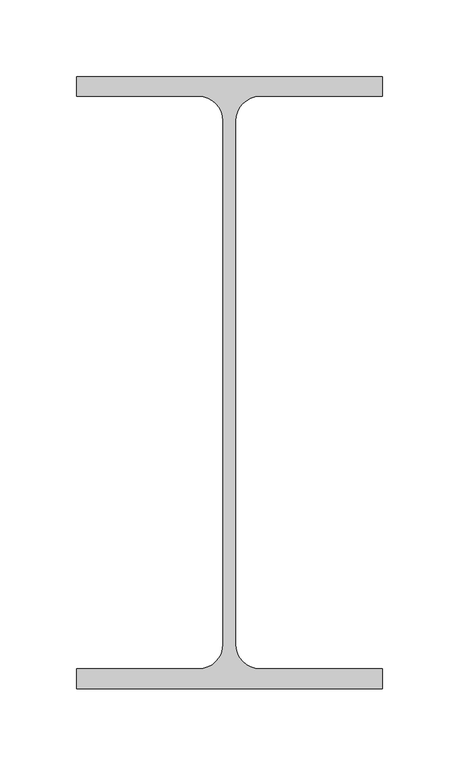
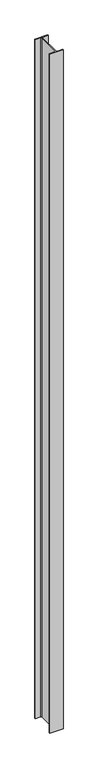
"""IFC4 building model written with IfcOpenShell, lengths in millimetres: column geometry, 0912_Steel Column_H_KSD3502 : H_SC_ASC_H-400x200x8x13."""

import ifcopenshell
import ifcopenshell.guid

model = None  # the IFC model being written
_history = None  # IfcOwnerHistory: only IFC2X3 demands one
_inside = {}  # id of a spatial element -> (the spatial element, [elements in it])
_under = {}  # id of a project, library or spatial element -> (it, [spatial elements below it])
_declared = {}  # id of a project -> (the project, [libraries it declares])
_typed = {}  # id of a type object -> (the type object, [elements of that type])
_made_of = {}  # id of a material, layer set ... -> (it, [elements and type objects made of it])


def new_model(schema):
    """Start an empty IFC model of exactly this schema.

    Asked for "IFC4X3", IfcOpenShell would pick the latest addendum, in which some entities
    have other attributes; the version numbers below select the first issue.
    IFC2X3 requires an IfcOwnerHistory on every rooted entity: one is made here for all.
    """
    global model, _history
    if schema == "IFC4X3":
        model = ifcopenshell.file(schema_version=(4, 3, 0, 0))
    else:
        model = ifcopenshell.file(schema=schema)
    _inside.clear()
    _under.clear()
    _declared.clear()
    _typed.clear()
    _made_of.clear()
    _history = None
    if model.schema == "IFC2X3":
        org = make("IfcOrganization", Name="unknown")
        user = make(
            "IfcPersonAndOrganization",
            ThePerson=make("IfcPerson", FamilyName="unknown"),
            TheOrganization=org,
        )
        app = make(
            "IfcApplication",
            ApplicationDeveloper=org,
            Version="unknown",
            ApplicationFullName="unknown",
            ApplicationIdentifier="unknown",
        )
        _history = make(
            "IfcOwnerHistory",
            OwningUser=user,
            OwningApplication=app,
            ChangeAction="ADDED",
            CreationDate=0,
        )
    return model


def make(cls, **values):
    """One entity of the class cls with the attributes given. An attribute that is None is left unset."""
    return model.create_entity(
        cls, **{name: value for name, value in values.items() if value is not None}
    )


def rooted(cls, **values):
    """An entity with a GlobalId (a new one), such as an element, a storey or a relation."""
    return make(cls, GlobalId=ifcopenshell.guid.new(), OwnerHistory=_history, **values)


def si_unit(unit_type, name, prefix=None):
    """IfcSIUnit, for example si_unit("LENGTHUNIT", "METRE", prefix="MILLI")."""
    return make("IfcSIUnit", UnitType=unit_type, Prefix=prefix, Name=name)


def assignment(units):
    """IfcUnitAssignment: the units of a project."""
    return None if units is None else make("IfcUnitAssignment", Units=units)


def point(xyz):
    """IfcCartesianPoint."""
    return None if xyz is None else make("IfcCartesianPoint", Coordinates=xyz)


def direction(xyz):
    """IfcDirection."""
    return None if xyz is None else make("IfcDirection", DirectionRatios=xyz)


def frame(location, z_axis=None, x_axis=None):
    """IfcAxis2Placement3D, a coordinate frame: its origin and axes. An axis left out is left unset."""
    return make(
        "IfcAxis2Placement3D",
        Location=point(location),
        Axis=direction(z_axis),
        RefDirection=direction(x_axis),
    )


def frame_2d(location, x_axis=None):
    """IfcAxis2Placement2D, a coordinate frame in the plane: its origin and x axis."""
    return make(
        "IfcAxis2Placement2D", Location=point(location), RefDirection=direction(x_axis)
    )


def origin():
    """The frame at (0, 0, 0) with its axes left unset."""
    return frame((0.0, 0.0, 0.0))


def place(relative_to, where):
    """IfcLocalPlacement: puts the frame where relative to a parent placement (None: the world)."""
    return make(
        "IfcLocalPlacement", PlacementRelTo=relative_to, RelativePlacement=where
    )


def context(
    kind, dimensions, precision=None, world=None, true_north=None, identifier=None
):
    """IfcGeometricRepresentationContext, for example the 3D "Model" context."""
    return make(
        "IfcGeometricRepresentationContext",
        ContextIdentifier=identifier,
        ContextType=kind,
        CoordinateSpaceDimension=dimensions,
        Precision=precision,
        WorldCoordinateSystem=world,
        TrueNorth=true_north,
    )


def project(units=None, contexts=None):
    """IfcProject with its units and contexts."""
    return rooted(
        "IfcProject",
        Name="project",
        RepresentationContexts=contexts,
        UnitsInContext=assignment(units),
    )


def spatial(cls, under=None, at=None, **own):
    """A site, building, storey or space (cls), placed at a placement, below another one or the project."""
    s = rooted(cls, ObjectPlacement=at, **own)
    if under is not None:
        _under.setdefault(under.id(), (under, []))[1].append(s)
    return s


def polyline(points):
    """IfcPolyline through the points."""
    return make("IfcPolyline", Points=[point(p) for p in points])


def circle_curve(where, radius):
    """IfcCircle in the frame where."""
    return make("IfcCircle", Position=where, Radius=radius)


def trimmed(basis, trim1, trim2, sense, master):
    """IfcTrimmedCurve: the piece of a basis curve between two trims."""
    return make(
        "IfcTrimmedCurve",
        BasisCurve=basis,
        Trim1=trim1,
        Trim2=trim2,
        SenseAgreement=sense,
        MasterRepresentation=master,
    )


def segment(curve, same_sense, transition):
    """IfcCompositeCurveSegment."""
    return make(
        "IfcCompositeCurveSegment",
        Transition=transition,
        SameSense=same_sense,
        ParentCurve=curve,
    )


def composite_curve(segments, self_intersect=None):
    """IfcCompositeCurve: segments joined end to end."""
    return make("IfcCompositeCurve", Segments=segments, SelfIntersect=self_intersect)


def outline(outer, holes=None, kind="AREA"):
    """IfcArbitraryClosedProfileDef: a profile drawn as a closed curve; with holes, ...WithVoids."""
    if holes is None:
        return make("IfcArbitraryClosedProfileDef", ProfileType=kind, OuterCurve=outer)
    return make(
        "IfcArbitraryProfileDefWithVoids",
        ProfileType=kind,
        OuterCurve=outer,
        InnerCurves=holes,
    )


def extrude(swept, where, along, depth):
    """IfcExtrudedAreaSolid: the profile swept, set in the frame where, extruded along a direction by depth."""
    return make(
        "IfcExtrudedAreaSolid",
        SweptArea=swept,
        Position=where,
        ExtrudedDirection=direction(along),
        Depth=depth,
    )


def shape(context_of_items, identifier, shape_type, items):
    """IfcShapeRepresentation: the items that make up one representation, for example the "Body"."""
    return make(
        "IfcShapeRepresentation",
        ContextOfItems=context_of_items,
        RepresentationIdentifier=identifier,
        RepresentationType=shape_type,
        Items=items,
    )


def source(mapping_origin, context_of_items, identifier, shape_type, items):
    """IfcRepresentationMap: a shape defined once, which mapped items show again and again."""
    return make(
        "IfcRepresentationMap",
        MappingOrigin=mapping_origin,
        MappedRepresentation=shape(context_of_items, identifier, shape_type, items),
    )


def transform(
    local_origin,
    x_axis=None,
    y_axis=None,
    z_axis=None,
    scale=None,
    scale2=None,
    scale3=None,
    uniform=True,
):
    """IfcCartesianTransformationOperator3D, or its non-uniform kind. x_axis, y_axis, z_axis: its Axis1, 2, 3."""
    if uniform:
        return make(
            "IfcCartesianTransformationOperator3D",
            Axis1=direction(x_axis),
            Axis2=direction(y_axis),
            LocalOrigin=point(local_origin),
            Scale=scale,
            Axis3=direction(z_axis),
        )
    return make(
        "IfcCartesianTransformationOperator3DnonUniform",
        Axis1=direction(x_axis),
        Axis2=direction(y_axis),
        LocalOrigin=point(local_origin),
        Scale=scale,
        Axis3=direction(z_axis),
        Scale2=scale2,
        Scale3=scale3,
    )


def mapped(mapping_source, mapping_target):
    """IfcMappedItem: shows the shape of a source again, moved by a transform."""
    return make(
        "IfcMappedItem", MappingSource=mapping_source, MappingTarget=mapping_target
    )


def made_of(thing, what):
    """Note that an element or type object is made of a material, layer set ...; save() writes the relation."""
    if what is not None:
        _made_of.setdefault(what.id(), (what, []))[1].append(thing)
    return thing


def element(
    cls,
    number,
    at=None,
    inside=None,
    cuts=None,
    type_object=None,
    material=None,
    context=None,
    identifier="Body",
    shape_type=None,
    held_by="IfcProductDefinitionShape",
    body=None,
    shapes=None,
    **own,
):
    """One element of the class cls, such as IfcWall. Its Tag is "e" and its number.

    at: its placement. inside: the storey or other place that contains it. cuts: it is an
    opening in that element (IfcRelVoidsElement). A single representation is given by context,
    identifier, shape_type and body (its items); several are given by shapes. held_by: the class
    of the entity that holds the representations. save() writes the other relations.
    """
    e = rooted(cls, Tag="e%d" % number, ObjectPlacement=at, **own)
    if body is not None:
        shapes = [shape(context, identifier, shape_type, body)]
    if shapes is not None:
        e.Representation = make(held_by, Representations=shapes)
    if inside is not None:
        _inside.setdefault(inside.id(), (inside, []))[1].append(e)
    if cuts is not None:
        rooted(
            "IfcRelVoidsElement", RelatingBuildingElement=cuts, RelatedOpeningElement=e
        )
    if type_object is not None:
        _typed.setdefault(type_object.id(), (type_object, []))[1].append(e)
    return made_of(e, material)


def aggregate(whole, parts):
    """IfcRelAggregates: a whole, such as a stair, and the parts it consists of."""
    return rooted("IfcRelAggregates", RelatingObject=whole, RelatedObjects=parts)


def save(model, path):
    """Write the relations noted so far, then the file.

    IfcRelAggregates (storeys below a building ...), IfcRelContainedInSpatialStructure (elements
    in a storey), IfcRelDefinesByType, IfcRelAssociatesMaterial and IfcRelDeclares: one each for
    every whole, place, type object, material and project.
    """
    for whole, parts in _under.values():
        aggregate(whole, parts)
    for where, things in _inside.values():
        rooted(
            "IfcRelContainedInSpatialStructure",
            RelatedElements=things,
            RelatingStructure=where,
        )
    for kind, things in _typed.values():
        rooted("IfcRelDefinesByType", RelatedObjects=things, RelatingType=kind)
    for what, things in _made_of.values():
        rooted("IfcRelAssociatesMaterial", RelatedObjects=things, RelatingMaterial=what)
    for by, libraries in _declared.values():
        rooted("IfcRelDeclares", RelatingContext=by, RelatedDefinitions=libraries)
    model.write(path)


def column_1d3624df(model_context):
    return source(origin(), model_context, "Body", "SweptSolid", [
        extrude(outline(composite_curve([segment(polyline([(100.0, 200.0), (100.0, 187.0), (20.0, 187.0)]), True, "CONTINUOUS"), segment(trimmed(circle_curve(frame_2d((20.0, 171.0)), 16.0), [point((20.0, 187.0))], [point((4.0, 171.0))], True, "CARTESIAN"), True, "CONTINUOUS"), segment(polyline([(4.0, 171.0), (4.0, -171.0)]), True, "CONTINUOUS"), segment(trimmed(circle_curve(frame_2d((20.0, -171.0)), 16.0), [point((4.0, -171.0))], [point((20.0, -187.0))], True, "CARTESIAN"), True, "CONTINUOUS"), segment(polyline([(20.0, -187.0), (100.0, -187.0), (100.0, -200.0), (-100.0, -200.0), (-100.0, -187.0), (-20.0, -187.0)]), True, "CONTINUOUS"), segment(trimmed(circle_curve(frame_2d((-20.0, -171.0)), 16.0), [point((-20.0, -187.0))], [point((-4.0, -171.0))], True, "CARTESIAN"), True, "CONTINUOUS"), segment(polyline([(-4.0, -171.0), (-4.0, 171.0)]), True, "CONTINUOUS"), segment(trimmed(circle_curve(frame_2d((-20.0, 171.0)), 16.0), [point((-4.0, 171.0))], [point((-20.0, 187.0))], True, "CARTESIAN"), True, "CONTINUOUS"), segment(polyline([(-20.0, 187.0), (-100.0, 187.0), (-100.0, 200.0), (100.0, 200.0)]), True, "CONTINUOUS")], self_intersect=False)), frame((0.0, 0.0, 6949.9720055), z_axis=(0.0, 0.0, 1.0), x_axis=(1.0, 0.0, 0.0)), (0.0, 0.0, 1.0), 11000.0),
    ])


if __name__ == "__main__":
    model = new_model("IFC4")
    model_context = context("Model", 3, world=origin())
    ifc_project = project(units=[si_unit("LENGTHUNIT", "METRE", prefix="MILLI")], contexts=[model_context])
    site = spatial("IfcSite", under=ifc_project)
    building = spatial("IfcBuilding", under=site)
    placement = place(None, origin())
    column_shape = column_1d3624df(model_context)
    element("IfcColumn", 1, ObjectType="0912_Steel Column_H_KSD3502 : H_SC_ASC_H-400x200x8x13", at=placement, inside=building, context=model_context, shape_type="MappedRepresentation", body=[
        mapped(column_shape, transform((0.0, 0.0, 0.0), x_axis=(1.0, 0.0, 0.0), y_axis=(0.0, 1.0, 0.0), z_axis=(0.0, 0.0, 1.0))),
    ])
    save(model, "model.ifc")

# Revit data of these elements
# Type "0912_Steel Column_H_KSD3502 : H_SC_ASC_H-400x200x8x13"
#   H_WM Code_1 = "S01AA002-00001 | Main Steel Structure Fabrication Work | Shelter/Building | Medium Steel - Standard (90KG/M>Weight≥30KG/M) | Material: (   )"
#   H_WM Code_2 = "S03AA028-00001 | Main Steel Structure Erection Work | Shelter/Building | Medium Steel (90KG/M>Weight≥30KG/M) | Material: (   )"
#   H_WM Code_3 = "S01AA010-00001 | Main Steel Structure Fabrication Work | Shelter/Building | Steel Painting/Coating | for Non-Fireproofed Steel Surface, Surface Preparation, Primer, Second & Final Coat | Material: (   )"
#   H_Q'ty Cal Type Tag = "SC-Q2"
#   Width = 20.0 cm
#   Web Thickness = 0.8 cm
#   Web Fillet = 1.6 cm
#   Warping Constant = 648999.0 cm⁶
#   Torsional Moment of Inertia = 35.8981 cm⁴
#   Section Area = 84.12 cm²
#   Plastic Modulus weak axis = 268.0 cm³
#   Plastic Modulus strong axis = 1330.0 cm³
#   Perimeter = 1.56 m²/m
#   Nominal Weight = 66.00 kgf/m
#   Moment of Inertia weak axis = 1740.00 cm⁴
#   Moment of Inertia strong axis = 23700.00 cm⁴
#   Height = 40.0 cm
#   Flange Thickness = 1.3 cm
#   Elastic Modulus weak axis = 174.0 cm³
#   Elastic Modulus strong axis = 1190.0 cm³
#   Centroid Vertical = 20.0 cm
#   Centroid Horizontal = 10.0 cm
#   Structural Material [instance default] = Steel, 45-345
#   Section Name Key = ""
#   Bolt Spacing = 0
#   Assembly Code = ""
# Element 1 (IfcColumn, "0912_Steel Column_H_KSD3502 : H_SC_ASC_H-400x200x8x13")
#   Structural Material = none
# Materials
#   "Steel, 45-345": class "Metal", colour RGB 189 187 185, transparency 0, Description = "Steel 345 MPa", Cost = 0
